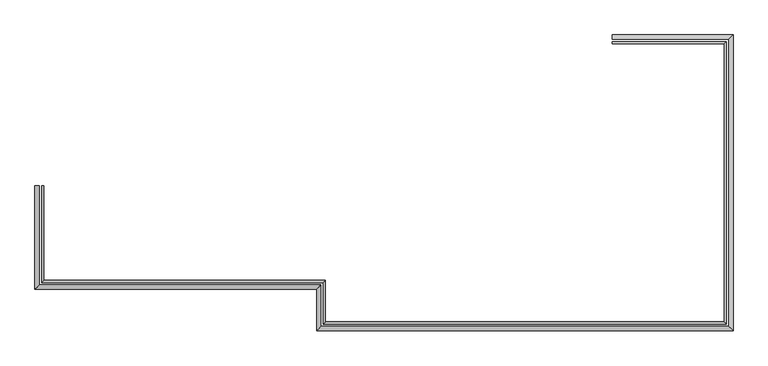
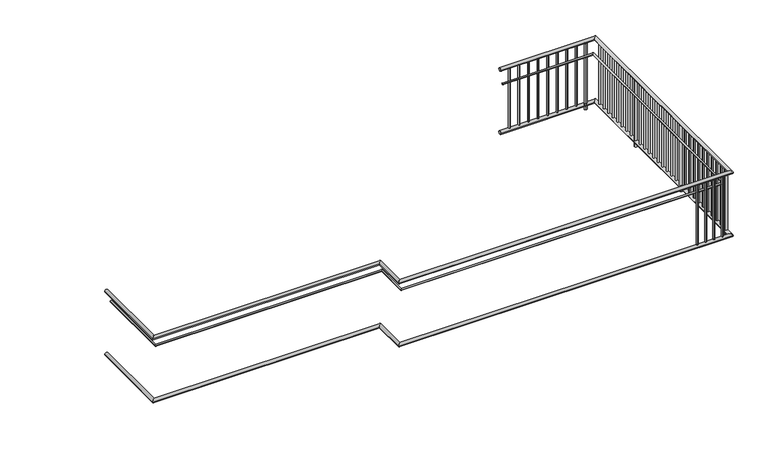
"""IFC4 building model written with IfcOpenShell, lengths in millimetres: railing geometry."""

import ifcopenshell
import ifcopenshell.guid

model = None  # the IFC model being written
_history = None  # IfcOwnerHistory: only IFC2X3 demands one
_inside = {}  # id of a spatial element -> (the spatial element, [elements in it])
_under = {}  # id of a project, library or spatial element -> (it, [spatial elements below it])
_declared = {}  # id of a project -> (the project, [libraries it declares])
_typed = {}  # id of a type object -> (the type object, [elements of that type])
_made_of = {}  # id of a material, layer set ... -> (it, [elements and type objects made of it])


def new_model(schema):
    """Start an empty IFC model of exactly this schema.

    Asked for "IFC4X3", IfcOpenShell would pick the latest addendum, in which some entities
    have other attributes; the version numbers below select the first issue.
    IFC2X3 requires an IfcOwnerHistory on every rooted entity: one is made here for all.
    """
    global model, _history
    if schema == "IFC4X3":
        model = ifcopenshell.file(schema_version=(4, 3, 0, 0))
    else:
        model = ifcopenshell.file(schema=schema)
    _inside.clear()
    _under.clear()
    _declared.clear()
    _typed.clear()
    _made_of.clear()
    _history = None
    if model.schema == "IFC2X3":
        org = make("IfcOrganization", Name="unknown")
        user = make(
            "IfcPersonAndOrganization",
            ThePerson=make("IfcPerson", FamilyName="unknown"),
            TheOrganization=org,
        )
        app = make(
            "IfcApplication",
            ApplicationDeveloper=org,
            Version="unknown",
            ApplicationFullName="unknown",
            ApplicationIdentifier="unknown",
        )
        _history = make(
            "IfcOwnerHistory",
            OwningUser=user,
            OwningApplication=app,
            ChangeAction="ADDED",
            CreationDate=0,
        )
    return model


def make(cls, **values):
    """One entity of the class cls with the attributes given. An attribute that is None is left unset."""
    return model.create_entity(
        cls, **{name: value for name, value in values.items() if value is not None}
    )


def rooted(cls, **values):
    """An entity with a GlobalId (a new one), such as an element, a storey or a relation."""
    return make(cls, GlobalId=ifcopenshell.guid.new(), OwnerHistory=_history, **values)


def si_unit(unit_type, name, prefix=None):
    """IfcSIUnit, for example si_unit("LENGTHUNIT", "METRE", prefix="MILLI")."""
    return make("IfcSIUnit", UnitType=unit_type, Prefix=prefix, Name=name)


def assignment(units):
    """IfcUnitAssignment: the units of a project."""
    return None if units is None else make("IfcUnitAssignment", Units=units)


def point(xyz):
    """IfcCartesianPoint."""
    return None if xyz is None else make("IfcCartesianPoint", Coordinates=xyz)


def direction(xyz):
    """IfcDirection."""
    return None if xyz is None else make("IfcDirection", DirectionRatios=xyz)


def frame(location, z_axis=None, x_axis=None):
    """IfcAxis2Placement3D, a coordinate frame: its origin and axes. An axis left out is left unset."""
    return make(
        "IfcAxis2Placement3D",
        Location=point(location),
        Axis=direction(z_axis),
        RefDirection=direction(x_axis),
    )


def frame_2d(location, x_axis=None):
    """IfcAxis2Placement2D, a coordinate frame in the plane: its origin and x axis."""
    return make(
        "IfcAxis2Placement2D", Location=point(location), RefDirection=direction(x_axis)
    )


def origin():
    """The frame at (0, 0, 0) with its axes left unset."""
    return frame((0.0, 0.0, 0.0))


def place(relative_to, where):
    """IfcLocalPlacement: puts the frame where relative to a parent placement (None: the world)."""
    return make(
        "IfcLocalPlacement", PlacementRelTo=relative_to, RelativePlacement=where
    )


def context(
    kind, dimensions, precision=None, world=None, true_north=None, identifier=None
):
    """IfcGeometricRepresentationContext, for example the 3D "Model" context."""
    return make(
        "IfcGeometricRepresentationContext",
        ContextIdentifier=identifier,
        ContextType=kind,
        CoordinateSpaceDimension=dimensions,
        Precision=precision,
        WorldCoordinateSystem=world,
        TrueNorth=true_north,
    )


def project(units=None, contexts=None):
    """IfcProject with its units and contexts."""
    return rooted(
        "IfcProject",
        Name="project",
        RepresentationContexts=contexts,
        UnitsInContext=assignment(units),
    )


def spatial(cls, under=None, at=None, **own):
    """A site, building, storey or space (cls), placed at a placement, below another one or the project."""
    s = rooted(cls, ObjectPlacement=at, **own)
    if under is not None:
        _under.setdefault(under.id(), (under, []))[1].append(s)
    return s


def circle_curve(where, radius):
    """IfcCircle in the frame where."""
    return make("IfcCircle", Position=where, Radius=radius)


def ellipse_curve(where, semi_axis1, semi_axis2):
    """IfcEllipse in the frame where."""
    return make(
        "IfcEllipse", Position=where, SemiAxis1=semi_axis1, SemiAxis2=semi_axis2
    )


def trimmed(basis, trim1, trim2, sense, master):
    """IfcTrimmedCurve: the piece of a basis curve between two trims."""
    return make(
        "IfcTrimmedCurve",
        BasisCurve=basis,
        Trim1=trim1,
        Trim2=trim2,
        SenseAgreement=sense,
        MasterRepresentation=master,
    )


def segment(curve, same_sense, transition):
    """IfcCompositeCurveSegment."""
    return make(
        "IfcCompositeCurveSegment",
        Transition=transition,
        SameSense=same_sense,
        ParentCurve=curve,
    )


def composite_curve(segments, self_intersect=None):
    """IfcCompositeCurve: segments joined end to end."""
    return make("IfcCompositeCurve", Segments=segments, SelfIntersect=self_intersect)


def outline(outer, holes=None, kind="AREA"):
    """IfcArbitraryClosedProfileDef: a profile drawn as a closed curve; with holes, ...WithVoids."""
    if holes is None:
        return make("IfcArbitraryClosedProfileDef", ProfileType=kind, OuterCurve=outer)
    return make(
        "IfcArbitraryProfileDefWithVoids",
        ProfileType=kind,
        OuterCurve=outer,
        InnerCurves=holes,
    )


def extrude(swept, where, along, depth):
    """IfcExtrudedAreaSolid: the profile swept, set in the frame where, extruded along a direction by depth."""
    return make(
        "IfcExtrudedAreaSolid",
        SweptArea=swept,
        Position=where,
        ExtrudedDirection=direction(along),
        Depth=depth,
    )


def shape(context_of_items, identifier, shape_type, items):
    """IfcShapeRepresentation: the items that make up one representation, for example the "Body"."""
    return make(
        "IfcShapeRepresentation",
        ContextOfItems=context_of_items,
        RepresentationIdentifier=identifier,
        RepresentationType=shape_type,
        Items=items,
    )


def source(mapping_origin, context_of_items, identifier, shape_type, items):
    """IfcRepresentationMap: a shape defined once, which mapped items show again and again."""
    return make(
        "IfcRepresentationMap",
        MappingOrigin=mapping_origin,
        MappedRepresentation=shape(context_of_items, identifier, shape_type, items),
    )


def transform(
    local_origin,
    x_axis=None,
    y_axis=None,
    z_axis=None,
    scale=None,
    scale2=None,
    scale3=None,
    uniform=True,
):
    """IfcCartesianTransformationOperator3D, or its non-uniform kind. x_axis, y_axis, z_axis: its Axis1, 2, 3."""
    if uniform:
        return make(
            "IfcCartesianTransformationOperator3D",
            Axis1=direction(x_axis),
            Axis2=direction(y_axis),
            LocalOrigin=point(local_origin),
            Scale=scale,
            Axis3=direction(z_axis),
        )
    return make(
        "IfcCartesianTransformationOperator3DnonUniform",
        Axis1=direction(x_axis),
        Axis2=direction(y_axis),
        LocalOrigin=point(local_origin),
        Scale=scale,
        Axis3=direction(z_axis),
        Scale2=scale2,
        Scale3=scale3,
    )


def mapped(mapping_source, mapping_target):
    """IfcMappedItem: shows the shape of a source again, moved by a transform."""
    return make(
        "IfcMappedItem", MappingSource=mapping_source, MappingTarget=mapping_target
    )


def made_of(thing, what):
    """Note that an element or type object is made of a material, layer set ...; save() writes the relation."""
    if what is not None:
        _made_of.setdefault(what.id(), (what, []))[1].append(thing)
    return thing


def element(
    cls,
    number,
    at=None,
    inside=None,
    cuts=None,
    type_object=None,
    material=None,
    context=None,
    identifier="Body",
    shape_type=None,
    held_by="IfcProductDefinitionShape",
    body=None,
    shapes=None,
    **own,
):
    """One element of the class cls, such as IfcWall. Its Tag is "e" and its number.

    at: its placement. inside: the storey or other place that contains it. cuts: it is an
    opening in that element (IfcRelVoidsElement). A single representation is given by context,
    identifier, shape_type and body (its items); several are given by shapes. held_by: the class
    of the entity that holds the representations. save() writes the other relations.
    """
    e = rooted(cls, Tag="e%d" % number, ObjectPlacement=at, **own)
    if body is not None:
        shapes = [shape(context, identifier, shape_type, body)]
    if shapes is not None:
        e.Representation = make(held_by, Representations=shapes)
    if inside is not None:
        _inside.setdefault(inside.id(), (inside, []))[1].append(e)
    if cuts is not None:
        rooted(
            "IfcRelVoidsElement", RelatingBuildingElement=cuts, RelatedOpeningElement=e
        )
    if type_object is not None:
        _typed.setdefault(type_object.id(), (type_object, []))[1].append(e)
    return made_of(e, material)


def aggregate(whole, parts):
    """IfcRelAggregates: a whole, such as a stair, and the parts it consists of."""
    return rooted("IfcRelAggregates", RelatingObject=whole, RelatedObjects=parts)


def save(model, path):
    """Write the relations noted so far, then the file.

    IfcRelAggregates (storeys below a building ...), IfcRelContainedInSpatialStructure (elements
    in a storey), IfcRelDefinesByType, IfcRelAssociatesMaterial and IfcRelDeclares: one each for
    every whole, place, type object, material and project.
    """
    for whole, parts in _under.values():
        aggregate(whole, parts)
    for where, things in _inside.values():
        rooted(
            "IfcRelContainedInSpatialStructure",
            RelatedElements=things,
            RelatingStructure=where,
        )
    for kind, things in _typed.values():
        rooted("IfcRelDefinesByType", RelatedObjects=things, RelatingType=kind)
    for what, things in _made_of.values():
        rooted("IfcRelAssociatesMaterial", RelatedObjects=things, RelatingMaterial=what)
    for by, libraries in _declared.values():
        rooted("IfcRelDeclares", RelatingContext=by, RelatedDefinitions=libraries)
    model.write(path)


def plane_surface(at):
    """IfcPlane: the flat surface through the origin of the frame at, square to its z axis."""
    return make("IfcPlane", Position=at)


def cylinder_surface(at, radius):
    """IfcCylindricalSurface: all points at the distance radius from the z axis of the frame at."""
    return make("IfcCylindricalSurface", Position=at, Radius=radius)


def advanced_brep(points, edges, surfaces, faces):
    """IfcAdvancedBrep: a solid bounded by faces that lie on surfaces and meet in shared edges.

    An edge is (start, end): straight between two places in points (the first is 0);
    or (start, end, curve); or (start, end, curve, False) where it runs against its curve.
    A face is (place in surfaces, loops), or (place, loops, False) where it looks against
    its surface's normal. A loop lists edges by number (the first is 1), with a minus sign
    where the edge is run from its end to its start. The first loop is the outer one.
    """
    corners = [point(p) for p in points]
    vertices = [make("IfcVertexPoint", VertexGeometry=c) for c in corners]
    made = []
    for start, end, *more in edges:
        made.append(
            make(
                "IfcEdgeCurve",
                EdgeStart=vertices[start],
                EdgeEnd=vertices[end],
                EdgeGeometry=more[0] if more else make("IfcPolyline", Points=[corners[start], corners[end]]),
                SameSense=more[1] if len(more) > 1 else True,
            )
        )
    hull = []
    for where, loops, *sense in faces:
        bounds = []
        for j, loop in enumerate(loops):
            ring = [make("IfcOrientedEdge", EdgeElement=made[abs(k) - 1], Orientation=k > 0) for k in loop]
            bounds.append(
                make(
                    "IfcFaceOuterBound" if j == 0 else "IfcFaceBound",
                    Bound=make("IfcEdgeLoop", EdgeList=ring),
                    Orientation=True,
                )
            )
        hull.append(make("IfcAdvancedFace", Bounds=bounds, FaceSurface=surfaces[where], SameSense=sense[0] if sense else True))
    return make("IfcAdvancedBrep", Outer=make("IfcClosedShell", CfsFaces=hull))


def railing_80b2a91e(model_context):
    return source(origin(), model_context, "Body", "SolidModel", [
        advanced_brep(
        [(-3300.274449, -6943.3965465, 4474.6), (-3249.474449, -6943.3965465, 4474.6), (-3249.474449, -8138.3965465, 4474.6), (-3300.274449, -8189.1965465, 4474.6), (144.725551, -8138.3965465, 4474.6), (93.925551, -8189.1965465, 4474.6), (144.725551, -8638.3965465, 4474.6), (93.925551, -8689.1965465, 4474.6), (5057.425551, -8638.3965465, 4474.6), (5108.225551, -8689.1965465, 4474.6), (5057.425551, -5178.2252792, 4474.6), (5108.225551, -5127.4252792, 4474.6), (3654.725551, -5127.4252792, 4474.6), (3654.725551, -5178.2252792, 4474.6)],
        [
            (0, 1, circle_curve(frame((-3274.874449, -6943.3965465, 4474.6), z_axis=(0.0, 1.0, 0.0), x_axis=(1.0, 0.0, 0.0)), 25.4)),
            (1, 0, circle_curve(frame((-3274.874449, -6943.3965465, 4474.6), z_axis=(0.0, 1.0, 0.0), x_axis=(1.0, 0.0, 0.0)), 25.4)),
            (1, 2),
            (2, 3, ellipse_curve(frame((-3274.874449, -8163.7965465, 4474.6), z_axis=(-0.7071067811865475, 0.7071067811865475, 0.0), x_axis=(0.7071067811865474, 0.7071067811865476, 0.0)), 35.9210245, 25.4)),
            (3, 0),
            (3, 2, ellipse_curve(frame((-3274.874449, -8163.7965465, 4474.6), z_axis=(-0.7071067811865475, 0.7071067811865475, 0.0), x_axis=(0.7071067811865474, 0.7071067811865476, 0.0)), 35.9210245, 25.4)),
            (2, 4),
            (4, 5, ellipse_curve(frame((119.325551, -8163.7965465, 4474.6), z_axis=(-0.7071067811865475, 0.7071067811865475, 0.0), x_axis=(-0.7071067811865476, -0.7071067811865474, 0.0)), 35.9210245, 25.4)),
            (5, 3),
            (5, 4, ellipse_curve(frame((119.325551, -8163.7965465, 4474.6), z_axis=(-0.7071067811865475, 0.7071067811865475, 0.0), x_axis=(-0.7071067811865476, -0.7071067811865474, 0.0)), 35.9210245, 25.4)),
            (4, 6),
            (6, 7, ellipse_curve(frame((119.325551, -8663.7965465, 4474.6), z_axis=(-0.7071067811865475, 0.7071067811865475, 0.0), x_axis=(0.7071067811865474, 0.7071067811865476, 0.0)), 35.9210245, 25.4)),
            (7, 5),
            (7, 6, ellipse_curve(frame((119.325551, -8663.7965465, 4474.6), z_axis=(-0.7071067811865475, 0.7071067811865475, 0.0), x_axis=(0.7071067811865474, 0.7071067811865476, 0.0)), 35.9210245, 25.4)),
            (6, 8),
            (8, 9, ellipse_curve(frame((5082.825551, -8663.7965465, 4474.6), z_axis=(-0.7071067811865475, -0.7071067811865475, 0.0), x_axis=(-0.7071067811865476, 0.7071067811865474, 0.0)), 35.9210245, 25.4)),
            (9, 7),
            (9, 8, ellipse_curve(frame((5082.825551, -8663.7965465, 4474.6), z_axis=(-0.7071067811865475, -0.7071067811865475, 0.0), x_axis=(-0.7071067811865476, 0.7071067811865474, 0.0)), 35.9210245, 25.4)),
            (8, 10),
            (10, 11, ellipse_curve(frame((5082.825551, -5152.8252792, 4474.6), z_axis=(0.7071067811865475, -0.7071067811865475, 0.0), x_axis=(-0.7071067811865474, -0.7071067811865476, 0.0)), 35.9210245, 25.4)),
            (11, 9),
            (11, 10, ellipse_curve(frame((5082.825551, -5152.8252792, 4474.6), z_axis=(0.7071067811865475, -0.7071067811865475, 0.0), x_axis=(-0.7071067811865474, -0.7071067811865476, 0.0)), 35.9210245, 25.4)),
            (12, 13, circle_curve(frame((3654.725551, -5152.8252792, 4474.6), z_axis=(-1.0, 0.0, 0.0), x_axis=(0.0, -1.0, 0.0)), 25.4)),
            (13, 12, circle_curve(frame((3654.725551, -5152.8252792, 4474.6), z_axis=(-1.0, 0.0, 0.0), x_axis=(0.0, -1.0, 0.0)), 25.4)),
            (10, 13),
            (12, 11),
        ],
        [
            plane_surface(frame((-3274.874449, -6943.3965465, 4500.0), z_axis=(0.0, 1.0, 0.0), x_axis=(0.0, 0.0, -1.0))),
            cylinder_surface(frame((-3274.874449, -6943.3965465, 4474.6), z_axis=(0.0, 1.0, 0.0), x_axis=(1.0, 0.0, 0.0)), 25.4),
            cylinder_surface(frame((-3274.874449, -8163.7965465, 4474.6), z_axis=(-1.0, 0.0, 0.0), x_axis=(0.0, 1.0, 0.0)), 25.4),
            cylinder_surface(frame((119.325551, -8163.7965465, 4474.6), z_axis=(0.0, 1.0, 0.0), x_axis=(1.0, 0.0, 0.0)), 25.4),
            cylinder_surface(frame((119.325551, -8663.7965465, 4474.6), z_axis=(-1.0, 0.0, 0.0), x_axis=(0.0, 1.0, 0.0)), 25.4),
            cylinder_surface(frame((5082.825551, -8663.7965465, 4474.6), z_axis=(0.0, -1.0, 0.0), x_axis=(-1.0, 0.0, 0.0)), 25.4),
            plane_surface(frame((3654.725551, -5152.8252792, 4500.0), z_axis=(-1.0, 0.0, 0.0), x_axis=(0.0, -1.0, 0.0))),
            cylinder_surface(frame((5082.825551, -5152.8252792, 4474.6), z_axis=(1.0, 0.0, 0.0), x_axis=(0.0, -1.0, 0.0)), 25.4),
        ],
        [
            (0, [[1, 2]]),
            (1, [[-2, 3, 4, 5]]),
            (1, [[-1, -5, 6, -3]]),
            (2, [[-4, 7, 8, 9]]),
            (2, [[-6, -9, 10, -7]]),
            (3, [[-8, 11, 12, 13]]),
            (3, [[-10, -13, 14, -11]]),
            (4, [[-12, 15, 16, 17]]),
            (4, [[-14, -17, 18, -15]]),
            (5, [[-16, 19, 20, 21]]),
            (5, [[-18, -21, 22, -19]]),
            (6, [[23, 24]]),
            (7, [[-20, 25, -23, 26]]),
            (7, [[-22, -26, -24, -25]]),
        ],
    ),
        advanced_brep(
        [(-3220.574449, -6943.3965465, 4287.3), (-3195.174449, -6943.3965465, 4287.3), (-3195.174449, -8084.0965465, 4287.3), (-3220.574449, -8109.4965465, 4287.3), (199.025551, -8084.0965465, 4287.3), (173.625551, -8109.4965465, 4287.3), (199.025551, -8584.0965465, 4287.3), (173.625551, -8609.4965465, 4287.3), (5003.125551, -8584.0965465, 4287.3), (5028.525551, -8609.4965465, 4287.3), (5003.125551, -5232.5252792, 4287.3), (5028.525551, -5207.1252792, 4287.3), (3654.725551, -5207.1252792, 4287.3), (3654.725551, -5232.5252792, 4287.3)],
        [
            (0, 1, circle_curve(frame((-3207.874449, -6943.3965465, 4287.3), z_axis=(0.0, 1.0, 0.0), x_axis=(1.0, 0.0, 0.0)), 12.7)),
            (1, 0, circle_curve(frame((-3207.874449, -6943.3965465, 4287.3), z_axis=(0.0, 1.0, 0.0), x_axis=(1.0, 0.0, 0.0)), 12.7)),
            (1, 2),
            (2, 3, ellipse_curve(frame((-3207.874449, -8096.7965465, 4287.3), z_axis=(-0.7071067811865475, 0.7071067811865475, 0.0), x_axis=(0.7071067811865474, 0.7071067811865476, 0.0)), 17.9605122, 12.7)),
            (3, 0),
            (3, 2, ellipse_curve(frame((-3207.874449, -8096.7965465, 4287.3), z_axis=(-0.7071067811865475, 0.7071067811865475, 0.0), x_axis=(0.7071067811865474, 0.7071067811865476, 0.0)), 17.9605122, 12.7)),
            (2, 4),
            (4, 5, ellipse_curve(frame((186.325551, -8096.7965465, 4287.3), z_axis=(-0.7071067811865475, 0.7071067811865475, 0.0), x_axis=(-0.7071067811865476, -0.7071067811865474, 0.0)), 17.9605122, 12.7)),
            (5, 3),
            (5, 4, ellipse_curve(frame((186.325551, -8096.7965465, 4287.3), z_axis=(-0.7071067811865475, 0.7071067811865475, 0.0), x_axis=(-0.7071067811865476, -0.7071067811865474, 0.0)), 17.9605122, 12.7)),
            (4, 6),
            (6, 7, ellipse_curve(frame((186.325551, -8596.7965465, 4287.3), z_axis=(-0.7071067811865475, 0.7071067811865475, 0.0), x_axis=(0.7071067811865474, 0.7071067811865476, 0.0)), 17.9605122, 12.7)),
            (7, 5),
            (7, 6, ellipse_curve(frame((186.325551, -8596.7965465, 4287.3), z_axis=(-0.7071067811865475, 0.7071067811865475, 0.0), x_axis=(0.7071067811865474, 0.7071067811865476, 0.0)), 17.9605122, 12.7)),
            (6, 8),
            (8, 9, ellipse_curve(frame((5015.825551, -8596.7965465, 4287.3), z_axis=(-0.7071067811865475, -0.7071067811865475, 0.0), x_axis=(-0.7071067811865476, 0.7071067811865474, 0.0)), 17.9605122, 12.7)),
            (9, 7),
            (9, 8, ellipse_curve(frame((5015.825551, -8596.7965465, 4287.3), z_axis=(-0.7071067811865475, -0.7071067811865475, 0.0), x_axis=(-0.7071067811865476, 0.7071067811865474, 0.0)), 17.9605122, 12.7)),
            (8, 10),
            (10, 11, ellipse_curve(frame((5015.825551, -5219.8252792, 4287.3), z_axis=(0.7071067811865475, -0.7071067811865475, 0.0), x_axis=(-0.7071067811865474, -0.7071067811865476, 0.0)), 17.9605122, 12.7)),
            (11, 9),
            (11, 10, ellipse_curve(frame((5015.825551, -5219.8252792, 4287.3), z_axis=(0.7071067811865475, -0.7071067811865475, 0.0), x_axis=(-0.7071067811865474, -0.7071067811865476, 0.0)), 17.9605122, 12.7)),
            (12, 13, circle_curve(frame((3654.725551, -5219.8252792, 4287.3), z_axis=(-1.0, 0.0, 0.0), x_axis=(0.0, -1.0, 0.0)), 12.7)),
            (13, 12, circle_curve(frame((3654.725551, -5219.8252792, 4287.3), z_axis=(-1.0, 0.0, 0.0), x_axis=(0.0, -1.0, 0.0)), 12.7)),
            (10, 13),
            (12, 11),
        ],
        [
            plane_surface(frame((-3207.874449, -6943.3965465, 4300.0), z_axis=(0.0, 1.0, 0.0), x_axis=(0.0, 0.0, -1.0))),
            cylinder_surface(frame((-3207.874449, -6943.3965465, 4287.3), z_axis=(0.0, 1.0, 0.0), x_axis=(1.0, 0.0, 0.0)), 12.7),
            cylinder_surface(frame((-3207.874449, -8096.7965465, 4287.3), z_axis=(-1.0, 0.0, 0.0), x_axis=(0.0, 1.0, 0.0)), 12.7),
            cylinder_surface(frame((186.325551, -8096.7965465, 4287.3), z_axis=(0.0, 1.0, 0.0), x_axis=(1.0, 0.0, 0.0)), 12.7),
            cylinder_surface(frame((186.325551, -8596.7965465, 4287.3), z_axis=(-1.0, 0.0, 0.0), x_axis=(0.0, 1.0, 0.0)), 12.7),
            cylinder_surface(frame((5015.825551, -8596.7965465, 4287.3), z_axis=(0.0, -1.0, 0.0), x_axis=(-1.0, 0.0, 0.0)), 12.7),
            plane_surface(frame((3654.725551, -5219.8252792, 4300.0), z_axis=(-1.0, 0.0, 0.0), x_axis=(0.0, -1.0, 0.0))),
            cylinder_surface(frame((5015.825551, -5219.8252792, 4287.3), z_axis=(1.0, 0.0, 0.0), x_axis=(0.0, -1.0, 0.0)), 12.7),
        ],
        [
            (0, [[1, 2]]),
            (1, [[-2, 3, 4, 5]]),
            (1, [[-1, -5, 6, -3]]),
            (2, [[-4, 7, 8, 9]]),
            (2, [[-6, -9, 10, -7]]),
            (3, [[-8, 11, 12, 13]]),
            (3, [[-10, -13, 14, -11]]),
            (4, [[-12, 15, 16, 17]]),
            (4, [[-14, -17, 18, -15]]),
            (5, [[-16, 19, 20, 21]]),
            (5, [[-18, -21, 22, -19]]),
            (6, [[23, 24]]),
            (7, [[-20, 25, -23, 26]]),
            (7, [[-22, -26, -24, -25]]),
        ],
    ),
        advanced_brep(
        [(-3300.274449, -6943.3965465, 3474.6), (-3249.474449, -6943.3965465, 3474.6), (-3249.474449, -8138.3965465, 3474.6), (-3300.274449, -8189.1965465, 3474.6), (144.725551, -8138.3965465, 3474.6), (93.925551, -8189.1965465, 3474.6), (144.725551, -8638.3965465, 3474.6), (93.925551, -8689.1965465, 3474.6), (5057.425551, -8638.3965465, 3474.6), (5108.225551, -8689.1965465, 3474.6), (5057.425551, -5178.2252792, 3474.6), (5108.225551, -5127.4252792, 3474.6), (3654.725551, -5127.4252792, 3474.6), (3654.725551, -5178.2252792, 3474.6)],
        [
            (0, 1, circle_curve(frame((-3274.874449, -6943.3965465, 3474.6), z_axis=(0.0, 1.0, 0.0), x_axis=(1.0, 0.0, 0.0)), 25.4)),
            (1, 0, circle_curve(frame((-3274.874449, -6943.3965465, 3474.6), z_axis=(0.0, 1.0, 0.0), x_axis=(1.0, 0.0, 0.0)), 25.4)),
            (1, 2),
            (2, 3, ellipse_curve(frame((-3274.874449, -8163.7965465, 3474.6), z_axis=(-0.7071067811865475, 0.7071067811865475, 0.0), x_axis=(0.7071067811865474, 0.7071067811865476, 0.0)), 35.9210245, 25.4)),
            (3, 0),
            (3, 2, ellipse_curve(frame((-3274.874449, -8163.7965465, 3474.6), z_axis=(-0.7071067811865475, 0.7071067811865475, 0.0), x_axis=(0.7071067811865474, 0.7071067811865476, 0.0)), 35.9210245, 25.4)),
            (2, 4),
            (4, 5, ellipse_curve(frame((119.325551, -8163.7965465, 3474.6), z_axis=(-0.7071067811865475, 0.7071067811865475, 0.0), x_axis=(-0.7071067811865476, -0.7071067811865474, 0.0)), 35.9210245, 25.4)),
            (5, 3),
            (5, 4, ellipse_curve(frame((119.325551, -8163.7965465, 3474.6), z_axis=(-0.7071067811865475, 0.7071067811865475, 0.0), x_axis=(-0.7071067811865476, -0.7071067811865474, 0.0)), 35.9210245, 25.4)),
            (4, 6),
            (6, 7, ellipse_curve(frame((119.325551, -8663.7965465, 3474.6), z_axis=(-0.7071067811865475, 0.7071067811865475, 0.0), x_axis=(0.7071067811865474, 0.7071067811865476, 0.0)), 35.9210245, 25.4)),
            (7, 5),
            (7, 6, ellipse_curve(frame((119.325551, -8663.7965465, 3474.6), z_axis=(-0.7071067811865475, 0.7071067811865475, 0.0), x_axis=(0.7071067811865474, 0.7071067811865476, 0.0)), 35.9210245, 25.4)),
            (6, 8),
            (8, 9, ellipse_curve(frame((5082.825551, -8663.7965465, 3474.6), z_axis=(-0.7071067811865475, -0.7071067811865475, 0.0), x_axis=(-0.7071067811865476, 0.7071067811865474, 0.0)), 35.9210245, 25.4)),
            (9, 7),
            (9, 8, ellipse_curve(frame((5082.825551, -8663.7965465, 3474.6), z_axis=(-0.7071067811865475, -0.7071067811865475, 0.0), x_axis=(-0.7071067811865476, 0.7071067811865474, 0.0)), 35.9210245, 25.4)),
            (8, 10),
            (10, 11, ellipse_curve(frame((5082.825551, -5152.8252792, 3474.6), z_axis=(0.7071067811865475, -0.7071067811865475, 0.0), x_axis=(-0.7071067811865474, -0.7071067811865476, 0.0)), 35.9210245, 25.4)),
            (11, 9),
            (11, 10, ellipse_curve(frame((5082.825551, -5152.8252792, 3474.6), z_axis=(0.7071067811865475, -0.7071067811865475, 0.0), x_axis=(-0.7071067811865474, -0.7071067811865476, 0.0)), 35.9210245, 25.4)),
            (12, 13, circle_curve(frame((3654.725551, -5152.8252792, 3474.6), z_axis=(-1.0, 0.0, 0.0), x_axis=(0.0, -1.0, 0.0)), 25.4)),
            (13, 12, circle_curve(frame((3654.725551, -5152.8252792, 3474.6), z_axis=(-1.0, 0.0, 0.0), x_axis=(0.0, -1.0, 0.0)), 25.4)),
            (10, 13),
            (12, 11),
        ],
        [
            plane_surface(frame((-3274.874449, -6943.3965465, 3500.0), z_axis=(0.0, 1.0, 0.0), x_axis=(0.0, 0.0, -1.0))),
            cylinder_surface(frame((-3274.874449, -6943.3965465, 3474.6), z_axis=(0.0, 1.0, 0.0), x_axis=(1.0, 0.0, 0.0)), 25.4),
            cylinder_surface(frame((-3274.874449, -8163.7965465, 3474.6), z_axis=(-1.0, 0.0, 0.0), x_axis=(0.0, 1.0, 0.0)), 25.4),
            cylinder_surface(frame((119.325551, -8163.7965465, 3474.6), z_axis=(0.0, 1.0, 0.0), x_axis=(1.0, 0.0, 0.0)), 25.4),
            cylinder_surface(frame((119.325551, -8663.7965465, 3474.6), z_axis=(-1.0, 0.0, 0.0), x_axis=(0.0, 1.0, 0.0)), 25.4),
            cylinder_surface(frame((5082.825551, -8663.7965465, 3474.6), z_axis=(0.0, -1.0, 0.0), x_axis=(-1.0, 0.0, 0.0)), 25.4),
            plane_surface(frame((3654.725551, -5152.8252792, 3500.0), z_axis=(-1.0, 0.0, 0.0), x_axis=(0.0, -1.0, 0.0))),
            cylinder_surface(frame((5082.825551, -5152.8252792, 3474.6), z_axis=(1.0, 0.0, 0.0), x_axis=(0.0, -1.0, 0.0)), 25.4),
        ],
        [
            (0, [[1, 2]]),
            (1, [[-2, 3, 4, 5]]),
            (1, [[-1, -5, 6, -3]]),
            (2, [[-4, 7, 8, 9]]),
            (2, [[-6, -9, 10, -7]]),
            (3, [[-8, 11, 12, 13]]),
            (3, [[-10, -13, 14, -11]]),
            (4, [[-12, 15, 16, 17]]),
            (4, [[-14, -17, 18, -15]]),
            (5, [[-16, 19, 20, 21]]),
            (5, [[-18, -21, 22, -19]]),
            (6, [[23, 24]]),
            (7, [[-20, 25, -23, 26]]),
            (7, [[-22, -26, -24, -25]]),
        ],
    ),
        extrude(outline(composite_curve([segment(trimmed(circle_curve(frame_2d((3797.535551, -5152.8252792)), 12.5), [point((3797.535551, -5140.3252792))], [point((3797.535551, -5165.3252792))], False, "CARTESIAN"), True, "CONTINUOUS"), segment(trimmed(circle_curve(frame_2d((3797.535551, -5152.8252792)), 12.5), [point((3797.535551, -5165.3252792))], [point((3797.535551, -5140.3252792))], False, "CARTESIAN"), True, "CONTINUOUS")], self_intersect=False)), frame((0.0, 0.0, 3500.0), z_axis=(0.0, 0.0, 1.0), x_axis=(1.0, 0.0, 0.0)), (0.0, 0.0, 1.0), 949.2),
        extrude(outline(composite_curve([segment(trimmed(circle_curve(frame_2d((3940.345551, -5152.8252792)), 12.5), [point((3940.345551, -5140.3252792))], [point((3940.345551, -5165.3252792))], False, "CARTESIAN"), True, "CONTINUOUS"), segment(trimmed(circle_curve(frame_2d((3940.345551, -5152.8252792)), 12.5), [point((3940.345551, -5165.3252792))], [point((3940.345551, -5140.3252792))], False, "CARTESIAN"), True, "CONTINUOUS")], self_intersect=False)), frame((0.0, 0.0, 3500.0), z_axis=(0.0, 0.0, 1.0), x_axis=(1.0, 0.0, 0.0)), (0.0, 0.0, 1.0), 949.2),
        extrude(outline(composite_curve([segment(trimmed(circle_curve(frame_2d((4083.155551, -5152.8252792)), 12.5), [point((4083.155551, -5140.3252792))], [point((4083.155551, -5165.3252792))], False, "CARTESIAN"), True, "CONTINUOUS"), segment(trimmed(circle_curve(frame_2d((4083.155551, -5152.8252792)), 12.5), [point((4083.155551, -5165.3252792))], [point((4083.155551, -5140.3252792))], False, "CARTESIAN"), True, "CONTINUOUS")], self_intersect=False)), frame((0.0, 0.0, 3500.0), z_axis=(0.0, 0.0, 1.0), x_axis=(1.0, 0.0, 0.0)), (0.0, 0.0, 1.0), 949.2),
        extrude(outline(composite_curve([segment(trimmed(circle_curve(frame_2d((4225.965551, -5152.8252792)), 12.5), [point((4225.965551, -5140.3252792))], [point((4225.965551, -5165.3252792))], False, "CARTESIAN"), True, "CONTINUOUS"), segment(trimmed(circle_curve(frame_2d((4225.965551, -5152.8252792)), 12.5), [point((4225.965551, -5165.3252792))], [point((4225.965551, -5140.3252792))], False, "CARTESIAN"), True, "CONTINUOUS")], self_intersect=False)), frame((0.0, 0.0, 3500.0), z_axis=(0.0, 0.0, 1.0), x_axis=(1.0, 0.0, 0.0)), (0.0, 0.0, 1.0), 949.2),
        extrude(outline(composite_curve([segment(trimmed(circle_curve(frame_2d((4368.775551, -5152.8252792)), 12.5), [point((4368.775551, -5140.3252792))], [point((4368.775551, -5165.3252792))], False, "CARTESIAN"), True, "CONTINUOUS"), segment(trimmed(circle_curve(frame_2d((4368.775551, -5152.8252792)), 12.5), [point((4368.775551, -5165.3252792))], [point((4368.775551, -5140.3252792))], False, "CARTESIAN"), True, "CONTINUOUS")], self_intersect=False)), frame((0.0, 0.0, 3500.0), z_axis=(0.0, 0.0, 1.0), x_axis=(1.0, 0.0, 0.0)), (0.0, 0.0, 1.0), 949.2),
        extrude(outline(composite_curve([segment(trimmed(circle_curve(frame_2d((4511.585551, -5152.8252792)), 12.5), [point((4511.585551, -5140.3252792))], [point((4511.585551, -5165.3252792))], False, "CARTESIAN"), True, "CONTINUOUS"), segment(trimmed(circle_curve(frame_2d((4511.585551, -5152.8252792)), 12.5), [point((4511.585551, -5165.3252792))], [point((4511.585551, -5140.3252792))], False, "CARTESIAN"), True, "CONTINUOUS")], self_intersect=False)), frame((0.0, 0.0, 3500.0), z_axis=(0.0, 0.0, 1.0), x_axis=(1.0, 0.0, 0.0)), (0.0, 0.0, 1.0), 949.2),
        extrude(outline(composite_curve([segment(trimmed(circle_curve(frame_2d((4654.395551, -5152.8252792)), 12.5), [point((4654.395551, -5140.3252792))], [point((4654.395551, -5165.3252792))], False, "CARTESIAN"), True, "CONTINUOUS"), segment(trimmed(circle_curve(frame_2d((4654.395551, -5152.8252792)), 12.5), [point((4654.395551, -5165.3252792))], [point((4654.395551, -5140.3252792))], False, "CARTESIAN"), True, "CONTINUOUS")], self_intersect=False)), frame((0.0, 0.0, 3500.0), z_axis=(0.0, 0.0, 1.0), x_axis=(1.0, 0.0, 0.0)), (0.0, 0.0, 1.0), 949.2),
        extrude(outline(composite_curve([segment(trimmed(circle_curve(frame_2d((4797.205551, -5152.8252792)), 12.5), [point((4797.205551, -5140.3252792))], [point((4797.205551, -5165.3252792))], False, "CARTESIAN"), True, "CONTINUOUS"), segment(trimmed(circle_curve(frame_2d((4797.205551, -5152.8252792)), 12.5), [point((4797.205551, -5165.3252792))], [point((4797.205551, -5140.3252792))], False, "CARTESIAN"), True, "CONTINUOUS")], self_intersect=False)), frame((0.0, 0.0, 3500.0), z_axis=(0.0, 0.0, 1.0), x_axis=(1.0, 0.0, 0.0)), (0.0, 0.0, 1.0), 949.2),
        extrude(outline(composite_curve([segment(trimmed(circle_curve(frame_2d((4940.015551, -5152.8252792)), 21.0), [point((4940.015551, -5131.8252792))], [point((4940.015551, -5173.8252792))], False, "CARTESIAN"), True, "CONTINUOUS"), segment(trimmed(circle_curve(frame_2d((4940.015551, -5152.8252792)), 21.0), [point((4940.015551, -5173.8252792))], [point((4940.015551, -5131.8252792))], False, "CARTESIAN"), True, "CONTINUOUS")], self_intersect=False)), frame((0.0, 0.0, 3400.0), z_axis=(0.0, 0.0, 1.0), x_axis=(1.0, 0.0, 0.0)), (0.0, 0.0, 1.0), 1049.2),
        extrude(outline(composite_curve([segment(trimmed(circle_curve(frame_2d((5082.825551, -5269.8576547)), 12.5), [point((5095.325551, -5269.8576547))], [point((5070.325551, -5269.8576547))], False, "CARTESIAN"), True, "CONTINUOUS"), segment(trimmed(circle_curve(frame_2d((5082.825551, -5269.8576547)), 12.5), [point((5070.325551, -5269.8576547))], [point((5095.325551, -5269.8576547))], False, "CARTESIAN"), True, "CONTINUOUS")], self_intersect=False)), frame((0.0, 0.0, 3500.0), z_axis=(0.0, 0.0, 1.0), x_axis=(1.0, 0.0, 0.0)), (0.0, 0.0, 1.0), 949.2),
        extrude(outline(composite_curve([segment(trimmed(circle_curve(frame_2d((5082.825551, -5386.8900303)), 12.5), [point((5095.325551, -5386.8900303))], [point((5070.325551, -5386.8900303))], False, "CARTESIAN"), True, "CONTINUOUS"), segment(trimmed(circle_curve(frame_2d((5082.825551, -5386.8900303)), 12.5), [point((5070.325551, -5386.8900303))], [point((5095.325551, -5386.8900303))], False, "CARTESIAN"), True, "CONTINUOUS")], self_intersect=False)), frame((0.0, 0.0, 3500.0), z_axis=(0.0, 0.0, 1.0), x_axis=(1.0, 0.0, 0.0)), (0.0, 0.0, 1.0), 949.2),
        extrude(outline(composite_curve([segment(trimmed(circle_curve(frame_2d((5082.825551, -5503.9224059)), 12.5), [point((5095.325551, -5503.9224059))], [point((5070.325551, -5503.9224059))], False, "CARTESIAN"), True, "CONTINUOUS"), segment(trimmed(circle_curve(frame_2d((5082.825551, -5503.9224059)), 12.5), [point((5070.325551, -5503.9224059))], [point((5095.325551, -5503.9224059))], False, "CARTESIAN"), True, "CONTINUOUS")], self_intersect=False)), frame((0.0, 0.0, 3500.0), z_axis=(0.0, 0.0, 1.0), x_axis=(1.0, 0.0, 0.0)), (0.0, 0.0, 1.0), 949.2),
        extrude(outline(composite_curve([segment(trimmed(circle_curve(frame_2d((5082.825551, -5620.9547815)), 12.5), [point((5095.325551, -5620.9547815))], [point((5070.325551, -5620.9547815))], False, "CARTESIAN"), True, "CONTINUOUS"), segment(trimmed(circle_curve(frame_2d((5082.825551, -5620.9547815)), 12.5), [point((5070.325551, -5620.9547815))], [point((5095.325551, -5620.9547815))], False, "CARTESIAN"), True, "CONTINUOUS")], self_intersect=False)), frame((0.0, 0.0, 3500.0), z_axis=(0.0, 0.0, 1.0), x_axis=(1.0, 0.0, 0.0)), (0.0, 0.0, 1.0), 949.2),
        extrude(outline(composite_curve([segment(trimmed(circle_curve(frame_2d((5082.825551, -5737.9871571)), 12.5), [point((5095.325551, -5737.9871571))], [point((5070.325551, -5737.9871571))], False, "CARTESIAN"), True, "CONTINUOUS"), segment(trimmed(circle_curve(frame_2d((5082.825551, -5737.9871571)), 12.5), [point((5070.325551, -5737.9871571))], [point((5095.325551, -5737.9871571))], False, "CARTESIAN"), True, "CONTINUOUS")], self_intersect=False)), frame((0.0, 0.0, 3500.0), z_axis=(0.0, 0.0, 1.0), x_axis=(1.0, 0.0, 0.0)), (0.0, 0.0, 1.0), 949.2),
        extrude(outline(composite_curve([segment(trimmed(circle_curve(frame_2d((5082.825551, -5855.0195326)), 12.5), [point((5095.325551, -5855.0195326))], [point((5070.325551, -5855.0195326))], False, "CARTESIAN"), True, "CONTINUOUS"), segment(trimmed(circle_curve(frame_2d((5082.825551, -5855.0195326)), 12.5), [point((5070.325551, -5855.0195326))], [point((5095.325551, -5855.0195326))], False, "CARTESIAN"), True, "CONTINUOUS")], self_intersect=False)), frame((0.0, 0.0, 3500.0), z_axis=(0.0, 0.0, 1.0), x_axis=(1.0, 0.0, 0.0)), (0.0, 0.0, 1.0), 949.2),
        extrude(outline(composite_curve([segment(trimmed(circle_curve(frame_2d((5082.825551, -5972.0519082)), 12.5), [point((5095.325551, -5972.0519082))], [point((5070.325551, -5972.0519082))], False, "CARTESIAN"), True, "CONTINUOUS"), segment(trimmed(circle_curve(frame_2d((5082.825551, -5972.0519082)), 12.5), [point((5070.325551, -5972.0519082))], [point((5095.325551, -5972.0519082))], False, "CARTESIAN"), True, "CONTINUOUS")], self_intersect=False)), frame((0.0, 0.0, 3500.0), z_axis=(0.0, 0.0, 1.0), x_axis=(1.0, 0.0, 0.0)), (0.0, 0.0, 1.0), 949.2),
        extrude(outline(composite_curve([segment(trimmed(circle_curve(frame_2d((5082.825551, -6089.0842838)), 12.5), [point((5095.325551, -6089.0842838))], [point((5070.325551, -6089.0842838))], False, "CARTESIAN"), True, "CONTINUOUS"), segment(trimmed(circle_curve(frame_2d((5082.825551, -6089.0842838)), 12.5), [point((5070.325551, -6089.0842838))], [point((5095.325551, -6089.0842838))], False, "CARTESIAN"), True, "CONTINUOUS")], self_intersect=False)), frame((0.0, 0.0, 3500.0), z_axis=(0.0, 0.0, 1.0), x_axis=(1.0, 0.0, 0.0)), (0.0, 0.0, 1.0), 949.2),
        extrude(outline(composite_curve([segment(trimmed(circle_curve(frame_2d((5082.825551, -6206.1166594)), 21.0), [point((5103.825551, -6206.1166594))], [point((5061.825551, -6206.1166594))], False, "CARTESIAN"), True, "CONTINUOUS"), segment(trimmed(circle_curve(frame_2d((5082.825551, -6206.1166594)), 21.0), [point((5061.825551, -6206.1166594))], [point((5103.825551, -6206.1166594))], False, "CARTESIAN"), True, "CONTINUOUS")], self_intersect=False)), frame((0.0, 0.0, 3400.0), z_axis=(0.0, 0.0, 1.0), x_axis=(1.0, 0.0, 0.0)), (0.0, 0.0, 1.0), 1049.2),
        extrude(outline(composite_curve([segment(trimmed(circle_curve(frame_2d((5082.825551, -6323.1490349)), 12.5), [point((5095.325551, -6323.1490349))], [point((5070.325551, -6323.1490349))], False, "CARTESIAN"), True, "CONTINUOUS"), segment(trimmed(circle_curve(frame_2d((5082.825551, -6323.1490349)), 12.5), [point((5070.325551, -6323.1490349))], [point((5095.325551, -6323.1490349))], False, "CARTESIAN"), True, "CONTINUOUS")], self_intersect=False)), frame((0.0, 0.0, 3500.0), z_axis=(0.0, 0.0, 1.0), x_axis=(1.0, 0.0, 0.0)), (0.0, 0.0, 1.0), 949.2),
        extrude(outline(composite_curve([segment(trimmed(circle_curve(frame_2d((5082.825551, -6440.1814105)), 12.5), [point((5095.325551, -6440.1814105))], [point((5070.325551, -6440.1814105))], False, "CARTESIAN"), True, "CONTINUOUS"), segment(trimmed(circle_curve(frame_2d((5082.825551, -6440.1814105)), 12.5), [point((5070.325551, -6440.1814105))], [point((5095.325551, -6440.1814105))], False, "CARTESIAN"), True, "CONTINUOUS")], self_intersect=False)), frame((0.0, 0.0, 3500.0), z_axis=(0.0, 0.0, 1.0), x_axis=(1.0, 0.0, 0.0)), (0.0, 0.0, 1.0), 949.2),
        extrude(outline(composite_curve([segment(trimmed(circle_curve(frame_2d((5082.825551, -6557.2137861)), 12.5), [point((5095.325551, -6557.2137861))], [point((5070.325551, -6557.2137861))], False, "CARTESIAN"), True, "CONTINUOUS"), segment(trimmed(circle_curve(frame_2d((5082.825551, -6557.2137861)), 12.5), [point((5070.325551, -6557.2137861))], [point((5095.325551, -6557.2137861))], False, "CARTESIAN"), True, "CONTINUOUS")], self_intersect=False)), frame((0.0, 0.0, 3500.0), z_axis=(0.0, 0.0, 1.0), x_axis=(1.0, 0.0, 0.0)), (0.0, 0.0, 1.0), 949.2),
        extrude(outline(composite_curve([segment(trimmed(circle_curve(frame_2d((5082.825551, -6674.2461617)), 12.5), [point((5095.325551, -6674.2461617))], [point((5070.325551, -6674.2461617))], False, "CARTESIAN"), True, "CONTINUOUS"), segment(trimmed(circle_curve(frame_2d((5082.825551, -6674.2461617)), 12.5), [point((5070.325551, -6674.2461617))], [point((5095.325551, -6674.2461617))], False, "CARTESIAN"), True, "CONTINUOUS")], self_intersect=False)), frame((0.0, 0.0, 3500.0), z_axis=(0.0, 0.0, 1.0), x_axis=(1.0, 0.0, 0.0)), (0.0, 0.0, 1.0), 949.2),
        extrude(outline(composite_curve([segment(trimmed(circle_curve(frame_2d((5082.825551, -6791.2785373)), 12.5), [point((5095.325551, -6791.2785373))], [point((5070.325551, -6791.2785373))], False, "CARTESIAN"), True, "CONTINUOUS"), segment(trimmed(circle_curve(frame_2d((5082.825551, -6791.2785373)), 12.5), [point((5070.325551, -6791.2785373))], [point((5095.325551, -6791.2785373))], False, "CARTESIAN"), True, "CONTINUOUS")], self_intersect=False)), frame((0.0, 0.0, 3500.0), z_axis=(0.0, 0.0, 1.0), x_axis=(1.0, 0.0, 0.0)), (0.0, 0.0, 1.0), 949.2),
        extrude(outline(composite_curve([segment(trimmed(circle_curve(frame_2d((5082.825551, -6908.3109128)), 12.5), [point((5095.325551, -6908.3109128))], [point((5070.325551, -6908.3109128))], False, "CARTESIAN"), True, "CONTINUOUS"), segment(trimmed(circle_curve(frame_2d((5082.825551, -6908.3109128)), 12.5), [point((5070.325551, -6908.3109128))], [point((5095.325551, -6908.3109128))], False, "CARTESIAN"), True, "CONTINUOUS")], self_intersect=False)), frame((0.0, 0.0, 3500.0), z_axis=(0.0, 0.0, 1.0), x_axis=(1.0, 0.0, 0.0)), (0.0, 0.0, 1.0), 949.2),
        extrude(outline(composite_curve([segment(trimmed(circle_curve(frame_2d((5082.825551, -7025.3432884)), 12.5), [point((5095.325551, -7025.3432884))], [point((5070.325551, -7025.3432884))], False, "CARTESIAN"), True, "CONTINUOUS"), segment(trimmed(circle_curve(frame_2d((5082.825551, -7025.3432884)), 12.5), [point((5070.325551, -7025.3432884))], [point((5095.325551, -7025.3432884))], False, "CARTESIAN"), True, "CONTINUOUS")], self_intersect=False)), frame((0.0, 0.0, 3500.0), z_axis=(0.0, 0.0, 1.0), x_axis=(1.0, 0.0, 0.0)), (0.0, 0.0, 1.0), 949.2),
        extrude(outline(composite_curve([segment(trimmed(circle_curve(frame_2d((5082.825551, -7142.375664)), 12.5), [point((5095.325551, -7142.375664))], [point((5070.325551, -7142.375664))], False, "CARTESIAN"), True, "CONTINUOUS"), segment(trimmed(circle_curve(frame_2d((5082.825551, -7142.375664)), 12.5), [point((5070.325551, -7142.375664))], [point((5095.325551, -7142.375664))], False, "CARTESIAN"), True, "CONTINUOUS")], self_intersect=False)), frame((0.0, 0.0, 3500.0), z_axis=(0.0, 0.0, 1.0), x_axis=(1.0, 0.0, 0.0)), (0.0, 0.0, 1.0), 949.2),
        extrude(outline(composite_curve([segment(trimmed(circle_curve(frame_2d((5082.825551, -7259.4080396)), 12.5), [point((5095.325551, -7259.4080396))], [point((5070.325551, -7259.4080396))], False, "CARTESIAN"), True, "CONTINUOUS"), segment(trimmed(circle_curve(frame_2d((5082.825551, -7259.4080396)), 12.5), [point((5070.325551, -7259.4080396))], [point((5095.325551, -7259.4080396))], False, "CARTESIAN"), True, "CONTINUOUS")], self_intersect=False)), frame((0.0, 0.0, 3500.0), z_axis=(0.0, 0.0, 1.0), x_axis=(1.0, 0.0, 0.0)), (0.0, 0.0, 1.0), 949.2),
        extrude(outline(composite_curve([segment(trimmed(circle_curve(frame_2d((5082.825551, -7376.4404152)), 21.0), [point((5103.825551, -7376.4404152))], [point((5061.825551, -7376.4404152))], False, "CARTESIAN"), True, "CONTINUOUS"), segment(trimmed(circle_curve(frame_2d((5082.825551, -7376.4404152)), 21.0), [point((5061.825551, -7376.4404152))], [point((5103.825551, -7376.4404152))], False, "CARTESIAN"), True, "CONTINUOUS")], self_intersect=False)), frame((0.0, 0.0, 3400.0), z_axis=(0.0, 0.0, 1.0), x_axis=(1.0, 0.0, 0.0)), (0.0, 0.0, 1.0), 1049.2),
        extrude(outline(composite_curve([segment(trimmed(circle_curve(frame_2d((5082.825551, -7493.4727907)), 12.5), [point((5095.325551, -7493.4727907))], [point((5070.325551, -7493.4727907))], False, "CARTESIAN"), True, "CONTINUOUS"), segment(trimmed(circle_curve(frame_2d((5082.825551, -7493.4727907)), 12.5), [point((5070.325551, -7493.4727907))], [point((5095.325551, -7493.4727907))], False, "CARTESIAN"), True, "CONTINUOUS")], self_intersect=False)), frame((0.0, 0.0, 3500.0), z_axis=(0.0, 0.0, 1.0), x_axis=(1.0, 0.0, 0.0)), (0.0, 0.0, 1.0), 949.2),
        extrude(outline(composite_curve([segment(trimmed(circle_curve(frame_2d((5082.825551, -7610.5051663)), 12.5), [point((5095.325551, -7610.5051663))], [point((5070.325551, -7610.5051663))], False, "CARTESIAN"), True, "CONTINUOUS"), segment(trimmed(circle_curve(frame_2d((5082.825551, -7610.5051663)), 12.5), [point((5070.325551, -7610.5051663))], [point((5095.325551, -7610.5051663))], False, "CARTESIAN"), True, "CONTINUOUS")], self_intersect=False)), frame((0.0, 0.0, 3500.0), z_axis=(0.0, 0.0, 1.0), x_axis=(1.0, 0.0, 0.0)), (0.0, 0.0, 1.0), 949.2),
        extrude(outline(composite_curve([segment(trimmed(circle_curve(frame_2d((5082.825551, -7727.5375419)), 12.5), [point((5095.325551, -7727.5375419))], [point((5070.325551, -7727.5375419))], False, "CARTESIAN"), True, "CONTINUOUS"), segment(trimmed(circle_curve(frame_2d((5082.825551, -7727.5375419)), 12.5), [point((5070.325551, -7727.5375419))], [point((5095.325551, -7727.5375419))], False, "CARTESIAN"), True, "CONTINUOUS")], self_intersect=False)), frame((0.0, 0.0, 3500.0), z_axis=(0.0, 0.0, 1.0), x_axis=(1.0, 0.0, 0.0)), (0.0, 0.0, 1.0), 949.2),
        extrude(outline(composite_curve([segment(trimmed(circle_curve(frame_2d((5082.825551, -7844.5699175)), 12.5), [point((5095.325551, -7844.5699175))], [point((5070.325551, -7844.5699175))], False, "CARTESIAN"), True, "CONTINUOUS"), segment(trimmed(circle_curve(frame_2d((5082.825551, -7844.5699175)), 12.5), [point((5070.325551, -7844.5699175))], [point((5095.325551, -7844.5699175))], False, "CARTESIAN"), True, "CONTINUOUS")], self_intersect=False)), frame((0.0, 0.0, 3500.0), z_axis=(0.0, 0.0, 1.0), x_axis=(1.0, 0.0, 0.0)), (0.0, 0.0, 1.0), 949.2),
        extrude(outline(composite_curve([segment(trimmed(circle_curve(frame_2d((5082.825551, -7961.6022931)), 12.5), [point((5095.325551, -7961.6022931))], [point((5070.325551, -7961.6022931))], False, "CARTESIAN"), True, "CONTINUOUS"), segment(trimmed(circle_curve(frame_2d((5082.825551, -7961.6022931)), 12.5), [point((5070.325551, -7961.6022931))], [point((5095.325551, -7961.6022931))], False, "CARTESIAN"), True, "CONTINUOUS")], self_intersect=False)), frame((0.0, 0.0, 3500.0), z_axis=(0.0, 0.0, 1.0), x_axis=(1.0, 0.0, 0.0)), (0.0, 0.0, 1.0), 949.2),
        extrude(outline(composite_curve([segment(trimmed(circle_curve(frame_2d((5082.825551, -8078.6346686)), 12.5), [point((5095.325551, -8078.6346686))], [point((5070.325551, -8078.6346686))], False, "CARTESIAN"), True, "CONTINUOUS"), segment(trimmed(circle_curve(frame_2d((5082.825551, -8078.6346686)), 12.5), [point((5070.325551, -8078.6346686))], [point((5095.325551, -8078.6346686))], False, "CARTESIAN"), True, "CONTINUOUS")], self_intersect=False)), frame((0.0, 0.0, 3500.0), z_axis=(0.0, 0.0, 1.0), x_axis=(1.0, 0.0, 0.0)), (0.0, 0.0, 1.0), 949.2),
        extrude(outline(composite_curve([segment(trimmed(circle_curve(frame_2d((5082.825551, -8195.6670442)), 12.5), [point((5095.325551, -8195.6670442))], [point((5070.325551, -8195.6670442))], False, "CARTESIAN"), True, "CONTINUOUS"), segment(trimmed(circle_curve(frame_2d((5082.825551, -8195.6670442)), 12.5), [point((5070.325551, -8195.6670442))], [point((5095.325551, -8195.6670442))], False, "CARTESIAN"), True, "CONTINUOUS")], self_intersect=False)), frame((0.0, 0.0, 3500.0), z_axis=(0.0, 0.0, 1.0), x_axis=(1.0, 0.0, 0.0)), (0.0, 0.0, 1.0), 949.2),
        extrude(outline(composite_curve([segment(trimmed(circle_curve(frame_2d((5082.825551, -8312.6994198)), 12.5), [point((5095.325551, -8312.6994198))], [point((5070.325551, -8312.6994198))], False, "CARTESIAN"), True, "CONTINUOUS"), segment(trimmed(circle_curve(frame_2d((5082.825551, -8312.6994198)), 12.5), [point((5070.325551, -8312.6994198))], [point((5095.325551, -8312.6994198))], False, "CARTESIAN"), True, "CONTINUOUS")], self_intersect=False)), frame((0.0, 0.0, 3500.0), z_axis=(0.0, 0.0, 1.0), x_axis=(1.0, 0.0, 0.0)), (0.0, 0.0, 1.0), 949.2),
        extrude(outline(composite_curve([segment(trimmed(circle_curve(frame_2d((5082.825551, -8429.7317954)), 12.5), [point((5095.325551, -8429.7317954))], [point((5070.325551, -8429.7317954))], False, "CARTESIAN"), True, "CONTINUOUS"), segment(trimmed(circle_curve(frame_2d((5082.825551, -8429.7317954)), 12.5), [point((5070.325551, -8429.7317954))], [point((5095.325551, -8429.7317954))], False, "CARTESIAN"), True, "CONTINUOUS")], self_intersect=False)), frame((0.0, 0.0, 3500.0), z_axis=(0.0, 0.0, 1.0), x_axis=(1.0, 0.0, 0.0)), (0.0, 0.0, 1.0), 949.2),
        extrude(outline(composite_curve([segment(trimmed(circle_curve(frame_2d((5082.825551, -8546.764171)), 21.0), [point((5103.825551, -8546.764171))], [point((5061.825551, -8546.764171))], False, "CARTESIAN"), True, "CONTINUOUS"), segment(trimmed(circle_curve(frame_2d((5082.825551, -8546.764171)), 21.0), [point((5061.825551, -8546.764171))], [point((5103.825551, -8546.764171))], False, "CARTESIAN"), True, "CONTINUOUS")], self_intersect=False)), frame((0.0, 0.0, 3400.0), z_axis=(0.0, 0.0, 1.0), x_axis=(1.0, 0.0, 0.0)), (0.0, 0.0, 1.0), 1049.2),
        extrude(outline(composite_curve([segment(trimmed(circle_curve(frame_2d((4958.738051, -8663.7965465)), 12.5), [point((4958.738051, -8676.2965465))], [point((4958.738051, -8651.2965465))], False, "CARTESIAN"), True, "CONTINUOUS"), segment(trimmed(circle_curve(frame_2d((4958.738051, -8663.7965465)), 12.5), [point((4958.738051, -8651.2965465))], [point((4958.738051, -8676.2965465))], False, "CARTESIAN"), True, "CONTINUOUS")], self_intersect=False)), frame((0.0, 0.0, 3500.0), z_axis=(0.0, 0.0, 1.0), x_axis=(1.0, 0.0, 0.0)), (0.0, 0.0, 1.0), 949.2),
        extrude(outline(composite_curve([segment(trimmed(circle_curve(frame_2d((4834.650551, -8663.7965465)), 12.5), [point((4834.650551, -8676.2965465))], [point((4834.650551, -8651.2965465))], False, "CARTESIAN"), True, "CONTINUOUS"), segment(trimmed(circle_curve(frame_2d((4834.650551, -8663.7965465)), 12.5), [point((4834.650551, -8651.2965465))], [point((4834.650551, -8676.2965465))], False, "CARTESIAN"), True, "CONTINUOUS")], self_intersect=False)), frame((0.0, 0.0, 3500.0), z_axis=(0.0, 0.0, 1.0), x_axis=(1.0, 0.0, 0.0)), (0.0, 0.0, 1.0), 949.2),
        extrude(outline(composite_curve([segment(trimmed(circle_curve(frame_2d((4710.563051, -8663.7965465)), 12.5), [point((4710.563051, -8676.2965465))], [point((4710.563051, -8651.2965465))], False, "CARTESIAN"), True, "CONTINUOUS"), segment(trimmed(circle_curve(frame_2d((4710.563051, -8663.7965465)), 12.5), [point((4710.563051, -8651.2965465))], [point((4710.563051, -8676.2965465))], False, "CARTESIAN"), True, "CONTINUOUS")], self_intersect=False)), frame((0.0, 0.0, 3500.0), z_axis=(0.0, 0.0, 1.0), x_axis=(1.0, 0.0, 0.0)), (0.0, 0.0, 1.0), 949.2),
        extrude(outline(composite_curve([segment(trimmed(circle_curve(frame_2d((4586.475551, -8663.7965465)), 12.5), [point((4586.475551, -8676.2965465))], [point((4586.475551, -8651.2965465))], False, "CARTESIAN"), True, "CONTINUOUS"), segment(trimmed(circle_curve(frame_2d((4586.475551, -8663.7965465)), 12.5), [point((4586.475551, -8651.2965465))], [point((4586.475551, -8676.2965465))], False, "CARTESIAN"), True, "CONTINUOUS")], self_intersect=False)), frame((0.0, 0.0, 3500.0), z_axis=(0.0, 0.0, 1.0), x_axis=(1.0, 0.0, 0.0)), (0.0, 0.0, 1.0), 949.2),
    ])


if __name__ == "__main__":
    model = new_model("IFC4")
    model_context = context("Model", 3, world=origin())
    ifc_project = project(units=[si_unit("LENGTHUNIT", "METRE", prefix="MILLI")], contexts=[model_context])
    site = spatial("IfcSite", under=ifc_project)
    building = spatial("IfcBuilding", under=site)
    placement = place(None, origin())
    railing_shape = railing_80b2a91e(model_context)
    element("IfcRailing", 1, at=placement, inside=building, context=model_context, shape_type="MappedRepresentation", body=[
        mapped(railing_shape, transform((0.0, 0.0, 0.0), x_axis=(1.0, 0.0, 0.0), y_axis=(0.0, 1.0, 0.0), z_axis=(0.0, 0.0, 1.0))),
    ])
    save(model, "model.ifc")

# Revit data of these elements
# Project information
#   Project Issue Date = "Data de emissão"
#   Project Status = "Status do projeto"
#   Client Name = "Proprietário"
#   Project Address = "Insira aqui o endereço"
#   Project Name = "Nome do projeto"
#   Project Number = "0001"
# Element 1 (IfcRailing)
#   Materials on its faces: "Ferro - Pintura Esmalte"
# Materials
#   "Ferro - Pintura Esmalte": class "Pintura", colour RGB 255 255 255, transparency 0, Cost = 0
